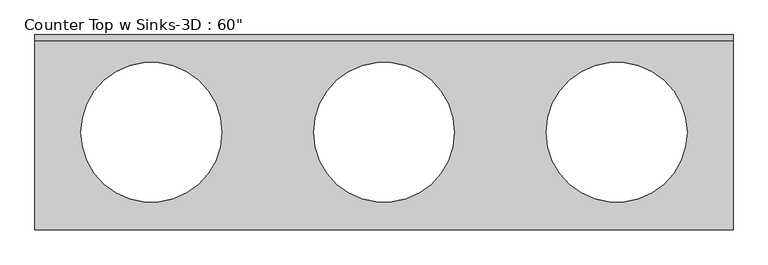
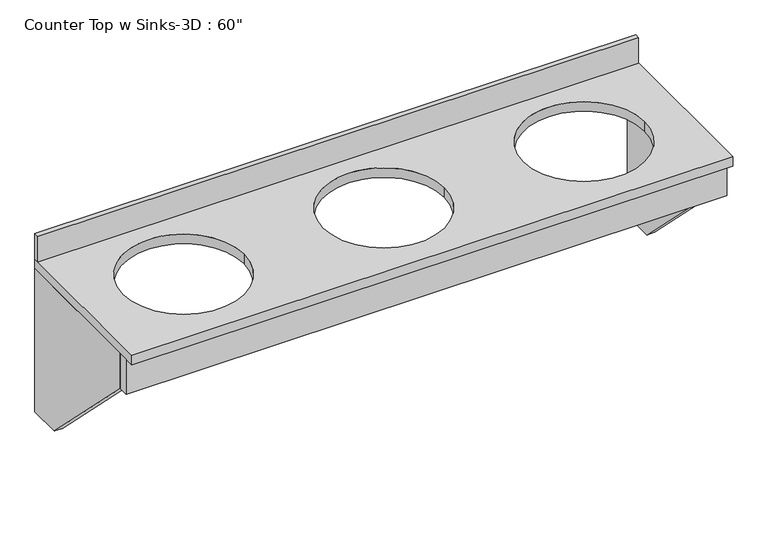
"""IFC4 building model written with IfcOpenShell, lengths in millimetres: furniture geometry."""

from ifc_helpers import new_model, si_unit, point, frame, frame_2d, origin, place, context, project, spatial, polyline, circle_curve, trimmed, segment, composite_curve, outline, extrude, source, transform, mapped, element, save


def furniture_ec8beb64(model_context):
    return source(origin(), model_context, "Body", "SweptSolid", [
        extrude(outline(polyline([(-198.4375, 825.5), (-198.4375, 254.0), (-325.4375, 254.0), (-757.2375, 685.8), (-757.2375, 825.5), (-198.4375, 825.5)])), frame((-1116.1103038, 0.0, 0.0), z_axis=(1.0, 0.0, 0.0), x_axis=(0.0, 1.0, 0.0)), (0.0, 0.0, 1.0), 31.75),
        extrude(outline(polyline([(-198.4375, 825.5), (-198.4375, 254.0), (-325.4375, 254.0), (-757.2375, 685.8), (-757.2375, 825.5), (-198.4375, 825.5)])), frame((1122.2646962, 0.0, 0.0), z_axis=(1.0, 0.0, 0.0), x_axis=(0.0, 1.0, 0.0)), (0.0, 0.0, 1.0), 31.75),
        extrude(outline(polyline([(-1116.1103038, -757.2375), (1154.0146962, -757.2375), (1154.0146962, -795.3375), (-1116.1103038, -795.3375), (-1116.1103038, -757.2375)])), frame((0.0, 0.0, 685.8), z_axis=(0.0, 0.0, 1.0), x_axis=(1.0, 0.0, 0.0)), (0.0, 0.0, 1.0), 139.7),
        extrude(outline(polyline([(1154.0146962, -198.4375), (1154.0146962, -217.4875), (-1116.1103038, -217.4875), (-1116.1103038, -198.4375), (1154.0146962, -198.4375)])), frame((0.0, 0.0, 863.6), z_axis=(0.0, 0.0, 1.0), x_axis=(1.0, 0.0, 0.0)), (0.0, 0.0, 1.0), 101.6),
        extrude(outline(polyline([(1154.0146962, -198.4375), (1154.0146962, -833.4375), (-1116.1103038, -833.4375), (-1116.1103038, -198.4375), (1154.0146962, -198.4375)]), holes=[composite_curve([segment(trimmed(circle_curve(frame_2d((-737.7561371, -515.9375)), 228.6), [point((-966.3561371, -515.9375))], [point((-509.1561371, -515.9375))], True, "CARTESIAN"), True, "CONTINUOUS"), segment(trimmed(circle_curve(frame_2d((-737.7561371, -515.9375)), 228.6), [point((-509.1561371, -515.9375))], [point((-966.3561371, -515.9375))], True, "CARTESIAN"), True, "CONTINUOUS")], self_intersect=False), composite_curve([segment(trimmed(circle_curve(frame_2d((775.6605295, -515.9375)), 228.6), [point((547.0605295, -515.9375))], [point((1004.2605295, -515.9375))], True, "CARTESIAN"), True, "CONTINUOUS"), segment(trimmed(circle_curve(frame_2d((775.6605295, -515.9375)), 228.6), [point((1004.2605295, -515.9375))], [point((547.0605295, -515.9375))], True, "CARTESIAN"), True, "CONTINUOUS")], self_intersect=False), composite_curve([segment(trimmed(circle_curve(frame_2d((18.9521962, -515.9375)), 228.6), [point((-209.6478038, -515.9375))], [point((247.5521962, -515.9375))], True, "CARTESIAN"), True, "CONTINUOUS"), segment(trimmed(circle_curve(frame_2d((18.9521962, -515.9375)), 228.6), [point((247.5521962, -515.9375))], [point((-209.6478038, -515.9375))], True, "CARTESIAN"), True, "CONTINUOUS")], self_intersect=False)]), frame((0.0, 0.0, 825.5), z_axis=(0.0, 0.0, 1.0), x_axis=(1.0, 0.0, 0.0)), (0.0, 0.0, 1.0), 38.1),
    ])


if __name__ == "__main__":
    model = new_model("IFC4")
    model_context = context("Model", 3, world=origin())
    ifc_project = project(units=[si_unit("LENGTHUNIT", "METRE", prefix="MILLI")], contexts=[model_context])
    site = spatial("IfcSite", under=ifc_project)
    building = spatial("IfcBuilding", under=site)
    placement = place(None, origin())
    furniture_shape = furniture_ec8beb64(model_context)
    element("IfcFurniture", 1, ObjectType="Counter Top w Sinks-3D : 60\"", at=placement, inside=building, context=model_context, shape_type="MappedRepresentation", body=[
        mapped(furniture_shape, transform((0.0, 0.0, 0.0), x_axis=(1.0, 0.0, 0.0), y_axis=(0.0, 1.0, 0.0), z_axis=(0.0, 0.0, 1.0))),
    ])
    save(model, "model.ifc")

# Revit data of these elements
# Type "Counter Top w Sinks-3D : 60\""
#   Assembly Code = "C1030400"
#   Height = 2' - 10"
#   Distance To Sink Center [instance default] = 1' - 3"
#   Clear Space = 2' - 3"
#   Counter Thickness = 0' - 1 1/2"
#   Depth = 2' - 1"
#   Length [instance default] = 5' - 0"
#   Number Of Sinks [instance default] = 2
#   Counter Top Material = Counter Top
#   Base Material = Laminate
#   Default Elevation = 0
# Element 1 (IfcFurniture, "Counter Top w Sinks-3D : 60\"")
#   Distance To Sink Center = 1' - 2.89583"
#   Length = 7' - 5 3/8"
#   Number Of Sinks = 3
#   Materials on its faces: "Counter Top", "Laminate"
# Materials
#   "Counter Top": class "Unassigned", colour RGB 247 247 239, transparency 0
#   "Laminate": class "Unassigned", colour RGB 247 235 201, transparency 0
